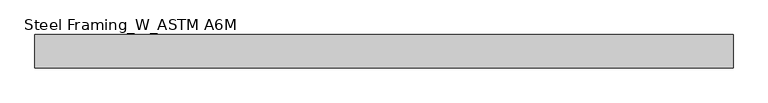
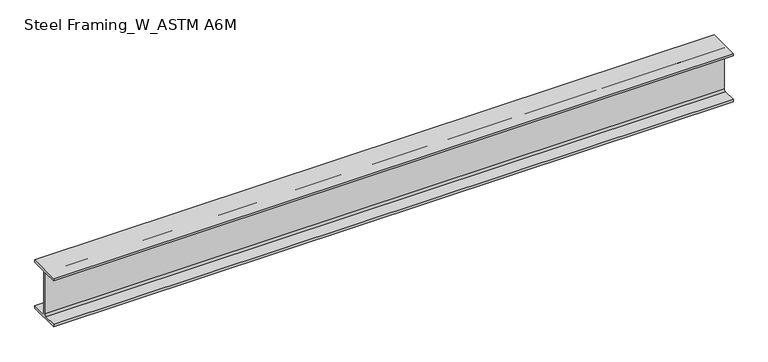
"""IFC4 building model written with IfcOpenShell, lengths in millimetres: beam geometry, Steel Framing_W_ASTM A6M : H_SB_AR_S02_W200x31.3_B6."""

from ifc_helpers import new_model, si_unit, point, frame, frame_2d, origin, place, context, project, spatial, polyline, circle_curve, trimmed, segment, composite_curve, outline, extrude, source, transform, mapped, element, save


def steel_framing_w_astm_a6m_5f95f2a9(model_context):
    return source(origin(), model_context, "Body", "SweptSolid", [
        extrude(outline(composite_curve([segment(polyline([(67.0, -94.8), (67.0, -105.0), (-67.0, -105.0), (-67.0, -94.8), (-10.775, -94.8)]), True, "CONTINUOUS"), segment(trimmed(circle_curve(frame_2d((-10.775, -87.2)), 7.6), [point((-10.775, -94.8))], [point((-3.175, -87.2))], True, "CARTESIAN"), True, "CONTINUOUS"), segment(polyline([(-3.175, -87.2), (-3.175, 87.2)]), True, "CONTINUOUS"), segment(trimmed(circle_curve(frame_2d((-10.775, 87.2)), 7.6), [point((-3.175, 87.2))], [point((-10.775, 94.8))], True, "CARTESIAN"), True, "CONTINUOUS"), segment(polyline([(-10.775, 94.8), (-67.0, 94.8), (-67.0, 105.0), (67.0, 105.0), (67.0, 94.8), (10.775, 94.8)]), True, "CONTINUOUS"), segment(trimmed(circle_curve(frame_2d((10.775, 87.2)), 7.6), [point((10.775, 94.8))], [point((3.175, 87.2))], True, "CARTESIAN"), True, "CONTINUOUS"), segment(polyline([(3.175, 87.2), (3.175, -87.2)]), True, "CONTINUOUS"), segment(trimmed(circle_curve(frame_2d((10.775, -87.2)), 7.6), [point((3.175, -87.2))], [point((10.775, -94.8))], True, "CARTESIAN"), True, "CONTINUOUS"), segment(polyline([(10.775, -94.8), (67.0, -94.8)]), True, "CONTINUOUS")], self_intersect=False)), frame((-1401.8, 0.0, 0.0), z_axis=(1.0, 0.0, 0.0), x_axis=(0.0, 1.0, 0.0)), (0.0, 0.0, 1.0), 2803.6),
    ])


if __name__ == "__main__":
    model = new_model("IFC4")
    model_context = context("Model", 3, world=origin())
    ifc_project = project(units=[si_unit("LENGTHUNIT", "METRE", prefix="MILLI")], contexts=[model_context])
    site = spatial("IfcSite", under=ifc_project)
    building = spatial("IfcBuilding", under=site)
    placement = place(None, origin())
    steel_framing_w_astm_a6m_shape = steel_framing_w_astm_a6m_5f95f2a9(model_context)
    element("IfcBeam", 1, ObjectType="Steel Framing_W_ASTM A6M : H_SB_AR_S02_W200x31.3_B6", at=placement, inside=building, context=model_context, shape_type="MappedRepresentation", body=[
        mapped(steel_framing_w_astm_a6m_shape, transform((0.0, 0.0, 0.0), x_axis=(1.0, 0.0, 0.0), y_axis=(0.0, 1.0, 0.0), z_axis=(0.0, 0.0, 1.0))),
    ])
    save(model, "model.ifc")

# Revit data of these elements
# Type "Steel Framing_W_ASTM A6M : H_SB_AR_S02_W200x31.3_B6"
#   Type Mark = "B6"
#   Section Name Key = "W8x21"
#   Width = 13.4 cm
#   Web Thickness = 0.635 cm
#   Web Fillet = 0.76 cm
#   Warping Constant = 40800.0 cm⁶
#   Torsional Moment of Inertia = 11.70 cm⁴
#   Section Area = 39.7 cm²
#   Plastic Modulus weak axis = 93.2 cm³
#   Plastic Modulus strong axis = 334.0 cm³
#   Perimeter = 0.93 m²/m
#   Nominal Weight = 31.30 kgf/m
#   Moment of Inertia weak axis = 407.00 cm⁴
#   Moment of Inertia strong axis = 3130.00 cm⁴
#   Height = 21.0 cm
#   Flange Thickness = 1.02 cm
#   Elastic Modulus weak axis = 60.8 cm³
#   Elastic Modulus strong axis = 298.0 cm³
#   Centroid Vertical = 10.5 cm
#   Centroid Horizontal = 6.7 cm
#   Length [instance default] = 1500 mm
#   Structural Material [instance default] = Steel, 45-345
#   Bolt Spacing = 0
#   Assembly Code = ""
# Element 1 (IfcBeam, "Steel Framing_W_ASTM A6M : H_SB_AR_S02_W200x31.3_B6")
#   Materials on its faces: "Steel, 45-345"
# Materials
#   "Steel, 45-345": class "Metal", colour RGB 189 187 185, transparency 0, Description = "Steel 345 MPa", Cost = 0
